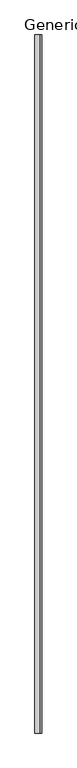
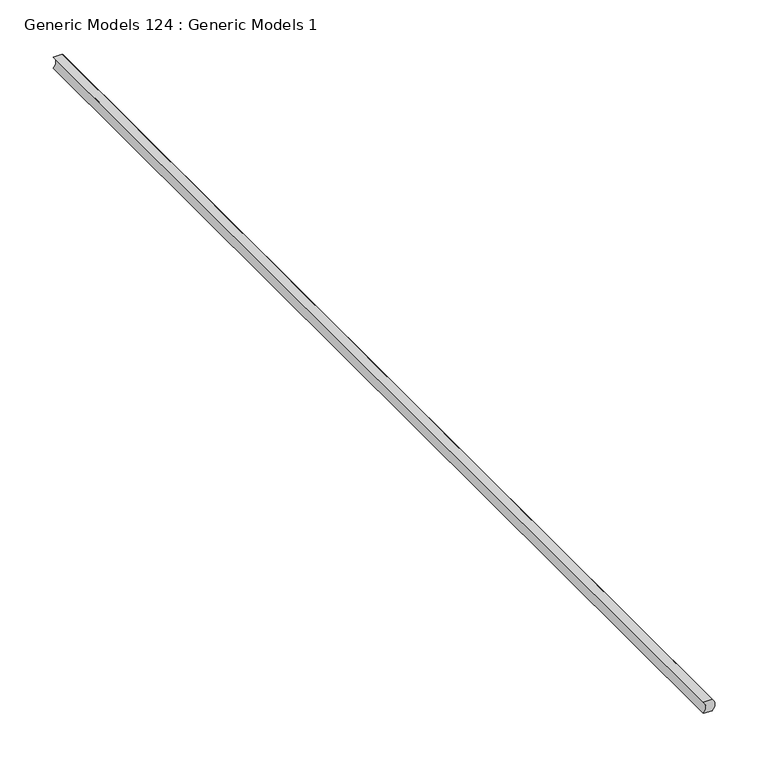
"""IFC4 building model written with IfcOpenShell, lengths in millimetres: proxy geometry, Generic Models 124 : Generic Models 1."""

import ifcopenshell
import ifcopenshell.guid

model = None  # the IFC model being written
_history = None  # IfcOwnerHistory: only IFC2X3 demands one
_inside = {}  # id of a spatial element -> (the spatial element, [elements in it])
_under = {}  # id of a project, library or spatial element -> (it, [spatial elements below it])
_declared = {}  # id of a project -> (the project, [libraries it declares])
_typed = {}  # id of a type object -> (the type object, [elements of that type])
_made_of = {}  # id of a material, layer set ... -> (it, [elements and type objects made of it])


def new_model(schema):
    """Start an empty IFC model of exactly this schema.

    Asked for "IFC4X3", IfcOpenShell would pick the latest addendum, in which some entities
    have other attributes; the version numbers below select the first issue.
    IFC2X3 requires an IfcOwnerHistory on every rooted entity: one is made here for all.
    """
    global model, _history
    if schema == "IFC4X3":
        model = ifcopenshell.file(schema_version=(4, 3, 0, 0))
    else:
        model = ifcopenshell.file(schema=schema)
    _inside.clear()
    _under.clear()
    _declared.clear()
    _typed.clear()
    _made_of.clear()
    _history = None
    if model.schema == "IFC2X3":
        org = make("IfcOrganization", Name="unknown")
        user = make(
            "IfcPersonAndOrganization",
            ThePerson=make("IfcPerson", FamilyName="unknown"),
            TheOrganization=org,
        )
        app = make(
            "IfcApplication",
            ApplicationDeveloper=org,
            Version="unknown",
            ApplicationFullName="unknown",
            ApplicationIdentifier="unknown",
        )
        _history = make(
            "IfcOwnerHistory",
            OwningUser=user,
            OwningApplication=app,
            ChangeAction="ADDED",
            CreationDate=0,
        )
    return model


def make(cls, **values):
    """One entity of the class cls with the attributes given. An attribute that is None is left unset."""
    return model.create_entity(
        cls, **{name: value for name, value in values.items() if value is not None}
    )


def rooted(cls, **values):
    """An entity with a GlobalId (a new one), such as an element, a storey or a relation."""
    return make(cls, GlobalId=ifcopenshell.guid.new(), OwnerHistory=_history, **values)


def si_unit(unit_type, name, prefix=None):
    """IfcSIUnit, for example si_unit("LENGTHUNIT", "METRE", prefix="MILLI")."""
    return make("IfcSIUnit", UnitType=unit_type, Prefix=prefix, Name=name)


def assignment(units):
    """IfcUnitAssignment: the units of a project."""
    return None if units is None else make("IfcUnitAssignment", Units=units)


def point(xyz):
    """IfcCartesianPoint."""
    return None if xyz is None else make("IfcCartesianPoint", Coordinates=xyz)


def direction(xyz):
    """IfcDirection."""
    return None if xyz is None else make("IfcDirection", DirectionRatios=xyz)


def frame(location, z_axis=None, x_axis=None):
    """IfcAxis2Placement3D, a coordinate frame: its origin and axes. An axis left out is left unset."""
    return make(
        "IfcAxis2Placement3D",
        Location=point(location),
        Axis=direction(z_axis),
        RefDirection=direction(x_axis),
    )


def frame_2d(location, x_axis=None):
    """IfcAxis2Placement2D, a coordinate frame in the plane: its origin and x axis."""
    return make(
        "IfcAxis2Placement2D", Location=point(location), RefDirection=direction(x_axis)
    )


def origin():
    """The frame at (0, 0, 0) with its axes left unset."""
    return frame((0.0, 0.0, 0.0))


def place(relative_to, where):
    """IfcLocalPlacement: puts the frame where relative to a parent placement (None: the world)."""
    return make(
        "IfcLocalPlacement", PlacementRelTo=relative_to, RelativePlacement=where
    )


def context(
    kind, dimensions, precision=None, world=None, true_north=None, identifier=None
):
    """IfcGeometricRepresentationContext, for example the 3D "Model" context."""
    return make(
        "IfcGeometricRepresentationContext",
        ContextIdentifier=identifier,
        ContextType=kind,
        CoordinateSpaceDimension=dimensions,
        Precision=precision,
        WorldCoordinateSystem=world,
        TrueNorth=true_north,
    )


def project(units=None, contexts=None):
    """IfcProject with its units and contexts."""
    return rooted(
        "IfcProject",
        Name="project",
        RepresentationContexts=contexts,
        UnitsInContext=assignment(units),
    )


def spatial(cls, under=None, at=None, **own):
    """A site, building, storey or space (cls), placed at a placement, below another one or the project."""
    s = rooted(cls, ObjectPlacement=at, **own)
    if under is not None:
        _under.setdefault(under.id(), (under, []))[1].append(s)
    return s


def polyline(points):
    """IfcPolyline through the points."""
    return make("IfcPolyline", Points=[point(p) for p in points])


def circle_curve(where, radius):
    """IfcCircle in the frame where."""
    return make("IfcCircle", Position=where, Radius=radius)


def trimmed(basis, trim1, trim2, sense, master):
    """IfcTrimmedCurve: the piece of a basis curve between two trims."""
    return make(
        "IfcTrimmedCurve",
        BasisCurve=basis,
        Trim1=trim1,
        Trim2=trim2,
        SenseAgreement=sense,
        MasterRepresentation=master,
    )


def segment(curve, same_sense, transition):
    """IfcCompositeCurveSegment."""
    return make(
        "IfcCompositeCurveSegment",
        Transition=transition,
        SameSense=same_sense,
        ParentCurve=curve,
    )


def composite_curve(segments, self_intersect=None):
    """IfcCompositeCurve: segments joined end to end."""
    return make("IfcCompositeCurve", Segments=segments, SelfIntersect=self_intersect)


def outline(outer, holes=None, kind="AREA"):
    """IfcArbitraryClosedProfileDef: a profile drawn as a closed curve; with holes, ...WithVoids."""
    if holes is None:
        return make("IfcArbitraryClosedProfileDef", ProfileType=kind, OuterCurve=outer)
    return make(
        "IfcArbitraryProfileDefWithVoids",
        ProfileType=kind,
        OuterCurve=outer,
        InnerCurves=holes,
    )


def extrude(swept, where, along, depth):
    """IfcExtrudedAreaSolid: the profile swept, set in the frame where, extruded along a direction by depth."""
    return make(
        "IfcExtrudedAreaSolid",
        SweptArea=swept,
        Position=where,
        ExtrudedDirection=direction(along),
        Depth=depth,
    )


def shape(context_of_items, identifier, shape_type, items):
    """IfcShapeRepresentation: the items that make up one representation, for example the "Body"."""
    return make(
        "IfcShapeRepresentation",
        ContextOfItems=context_of_items,
        RepresentationIdentifier=identifier,
        RepresentationType=shape_type,
        Items=items,
    )


def source(mapping_origin, context_of_items, identifier, shape_type, items):
    """IfcRepresentationMap: a shape defined once, which mapped items show again and again."""
    return make(
        "IfcRepresentationMap",
        MappingOrigin=mapping_origin,
        MappedRepresentation=shape(context_of_items, identifier, shape_type, items),
    )


def transform(
    local_origin,
    x_axis=None,
    y_axis=None,
    z_axis=None,
    scale=None,
    scale2=None,
    scale3=None,
    uniform=True,
):
    """IfcCartesianTransformationOperator3D, or its non-uniform kind. x_axis, y_axis, z_axis: its Axis1, 2, 3."""
    if uniform:
        return make(
            "IfcCartesianTransformationOperator3D",
            Axis1=direction(x_axis),
            Axis2=direction(y_axis),
            LocalOrigin=point(local_origin),
            Scale=scale,
            Axis3=direction(z_axis),
        )
    return make(
        "IfcCartesianTransformationOperator3DnonUniform",
        Axis1=direction(x_axis),
        Axis2=direction(y_axis),
        LocalOrigin=point(local_origin),
        Scale=scale,
        Axis3=direction(z_axis),
        Scale2=scale2,
        Scale3=scale3,
    )


def mapped(mapping_source, mapping_target):
    """IfcMappedItem: shows the shape of a source again, moved by a transform."""
    return make(
        "IfcMappedItem", MappingSource=mapping_source, MappingTarget=mapping_target
    )


def made_of(thing, what):
    """Note that an element or type object is made of a material, layer set ...; save() writes the relation."""
    if what is not None:
        _made_of.setdefault(what.id(), (what, []))[1].append(thing)
    return thing


def element(
    cls,
    number,
    at=None,
    inside=None,
    cuts=None,
    type_object=None,
    material=None,
    context=None,
    identifier="Body",
    shape_type=None,
    held_by="IfcProductDefinitionShape",
    body=None,
    shapes=None,
    **own,
):
    """One element of the class cls, such as IfcWall. Its Tag is "e" and its number.

    at: its placement. inside: the storey or other place that contains it. cuts: it is an
    opening in that element (IfcRelVoidsElement). A single representation is given by context,
    identifier, shape_type and body (its items); several are given by shapes. held_by: the class
    of the entity that holds the representations. save() writes the other relations.
    """
    e = rooted(cls, Tag="e%d" % number, ObjectPlacement=at, **own)
    if body is not None:
        shapes = [shape(context, identifier, shape_type, body)]
    if shapes is not None:
        e.Representation = make(held_by, Representations=shapes)
    if inside is not None:
        _inside.setdefault(inside.id(), (inside, []))[1].append(e)
    if cuts is not None:
        rooted(
            "IfcRelVoidsElement", RelatingBuildingElement=cuts, RelatedOpeningElement=e
        )
    if type_object is not None:
        _typed.setdefault(type_object.id(), (type_object, []))[1].append(e)
    return made_of(e, material)


def aggregate(whole, parts):
    """IfcRelAggregates: a whole, such as a stair, and the parts it consists of."""
    return rooted("IfcRelAggregates", RelatingObject=whole, RelatedObjects=parts)


def save(model, path):
    """Write the relations noted so far, then the file.

    IfcRelAggregates (storeys below a building ...), IfcRelContainedInSpatialStructure (elements
    in a storey), IfcRelDefinesByType, IfcRelAssociatesMaterial and IfcRelDeclares: one each for
    every whole, place, type object, material and project.
    """
    for whole, parts in _under.values():
        aggregate(whole, parts)
    for where, things in _inside.values():
        rooted(
            "IfcRelContainedInSpatialStructure",
            RelatedElements=things,
            RelatingStructure=where,
        )
    for kind, things in _typed.values():
        rooted("IfcRelDefinesByType", RelatedObjects=things, RelatingType=kind)
    for what, things in _made_of.values():
        rooted("IfcRelAssociatesMaterial", RelatedObjects=things, RelatingMaterial=what)
    for by, libraries in _declared.values():
        rooted("IfcRelDeclares", RelatingContext=by, RelatedDefinitions=libraries)
    model.write(path)


def generic_models_124_generic_models_1_b386a220(model_context):
    return source(origin(), model_context, "Body", "SweptSolid", [
        extrude(outline(composite_curve([segment(polyline([(2218.773933, 49246.8544263), (2218.773933, 49256.3794263)]), True, "CONTINUOUS"), segment(trimmed(circle_curve(frame_2d((2225.123933, 49250.5499453)), 8.620055), [point((2218.773933, 49256.3794263))], [point((2231.473933, 49256.3794263))], False, "CARTESIAN"), True, "CONTINUOUS"), segment(polyline([(2231.473933, 49256.3794263), (2231.473933, 49246.8544263)]), True, "CONTINUOUS"), segment(trimmed(circle_curve(frame_2d((2225.123933, 49241.0249453)), 8.620055), [point((2231.473933, 49246.8544263))], [point((2218.773933, 49246.8544263))], True, "CARTESIAN"), True, "CONTINUOUS")], self_intersect=False)), frame((0.0, 0.0, 0.0), z_axis=(0.0, 1.0, 0.0), x_axis=(0.0, 0.0, 1.0)), (0.0, 0.0, 1.0), 1219.2),
    ])


if __name__ == "__main__":
    model = new_model("IFC4")
    model_context = context("Model", 3, world=origin())
    ifc_project = project(units=[si_unit("LENGTHUNIT", "METRE", prefix="MILLI")], contexts=[model_context])
    site = spatial("IfcSite", under=ifc_project)
    building = spatial("IfcBuilding", under=site)
    placement = place(None, origin())
    generic_models_124_generic_models_1_shape = generic_models_124_generic_models_1_b386a220(model_context)
    element("IfcBuildingElementProxy", 1, Name="Generic Models 124 : Generic Models 1", ObjectType="Generic Models 124 : Generic Models 1", at=placement, inside=building, context=model_context, shape_type="MappedRepresentation", body=[
        mapped(generic_models_124_generic_models_1_shape, transform((0.0, 0.0, 0.0), x_axis=(1.0, 0.0, 0.0), y_axis=(0.0, 1.0, 0.0), z_axis=(0.0, 0.0, 1.0))),
    ])
    save(model, "model.ifc")

# Revit data of these elements
# Element 1 (IfcBuildingElementProxy, "Generic Models 124 : Generic Models 1")
#   Materials on its faces: "SEALANT (W/ BACKER ROD IF NECESSARY)"
# Materials
#   "SEALANT (W/ BACKER ROD IF NECESSARY)": class "Unassigned", colour RGB 120 120 120, transparency 0, Cost = 0
